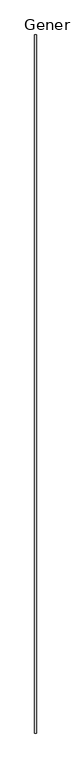
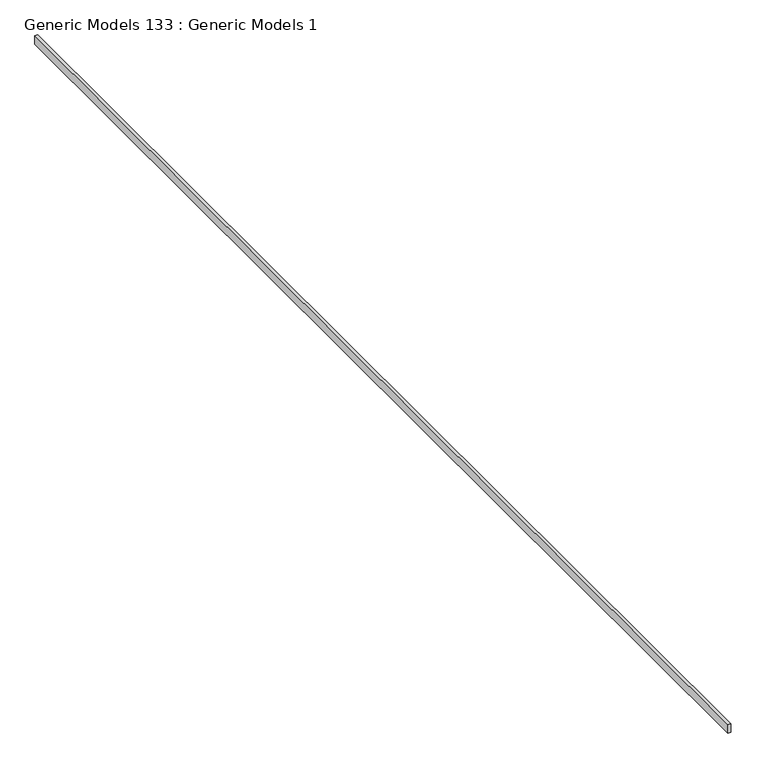
"""IFC4 building model written with IfcOpenShell, lengths in millimetres: proxy geometry, Generic Models 133 : Generic Models 1."""

from ifc_helpers import new_model, si_unit, frame, origin, place, context, project, spatial, polyline, outline, extrude, source, transform, mapped, element, save


def generic_models_133_generic_models_1_7b5242c6(model_context):
    return source(origin(), model_context, "Body", "SweptSolid", [
        extrude(outline(polyline([(7095.9513704, 11981.8769662), (7140.4013704, 11981.8769662), (7140.4013704, -7068.1230338), (7095.9513704, -7068.1230338), (7095.9513704, 11981.8769662)])), frame((0.0, 0.0, 126345.696), z_axis=(0.0, 0.0, 1.0), x_axis=(1.0, 0.0, 0.0)), (0.0, 0.0, 1.0), 139.7),
    ])


if __name__ == "__main__":
    model = new_model("IFC4")
    model_context = context("Model", 3, world=origin())
    ifc_project = project(units=[si_unit("LENGTHUNIT", "METRE", prefix="MILLI")], contexts=[model_context])
    site = spatial("IfcSite", under=ifc_project)
    building = spatial("IfcBuilding", under=site)
    placement = place(None, origin())
    generic_models_133_generic_models_1_shape = generic_models_133_generic_models_1_7b5242c6(model_context)
    element("IfcBuildingElementProxy", 1, Name="Generic Models 133 : Generic Models 1", ObjectType="Generic Models 133 : Generic Models 1", at=placement, inside=building, context=model_context, shape_type="MappedRepresentation", body=[
        mapped(generic_models_133_generic_models_1_shape, transform((0.0, 0.0, 0.0), x_axis=(1.0, 0.0, 0.0), y_axis=(0.0, 1.0, 0.0), z_axis=(0.0, 0.0, 1.0))),
    ])
    save(model, "model.ifc")

# Revit data of these elements
# Element 1 (IfcBuildingElementProxy, "Generic Models 133 : Generic Models 1")
#   Materials on its faces: "_STRUCTURAL MEMBER (SEE STRUCT. DWGS)"
# Materials
#   "_STRUCTURAL MEMBER (SEE STRUCT. DWGS)": class "Generic", colour RGB 209 182 141, transparency 0, Cost = 0
